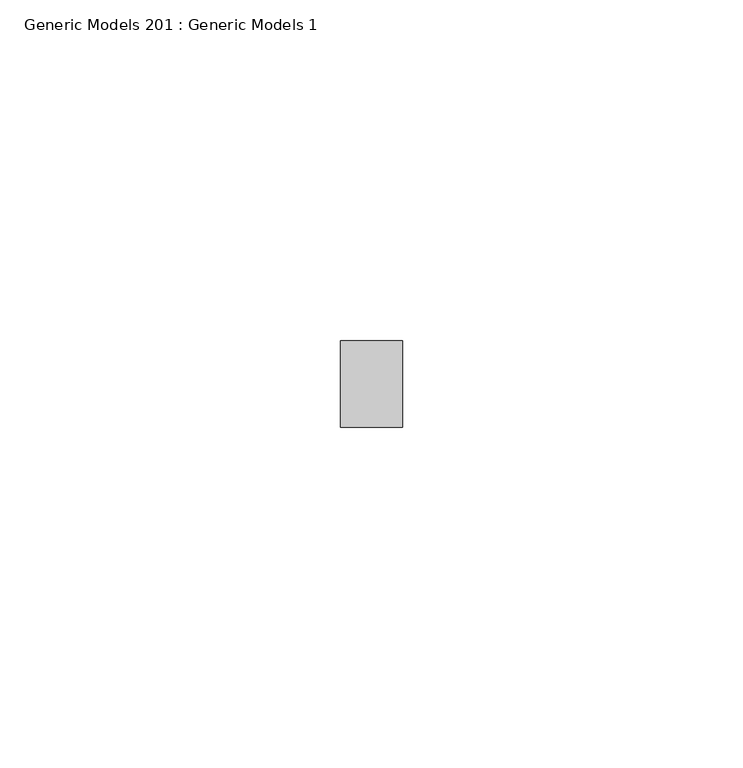
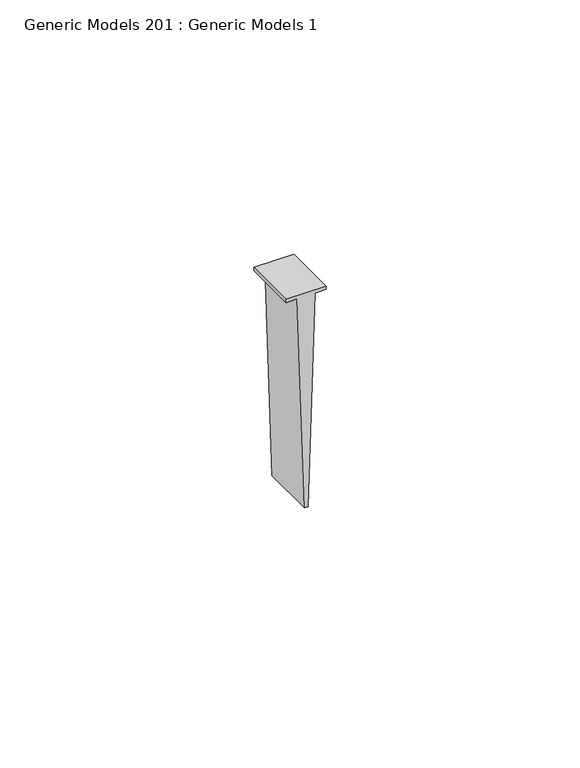
"""IFC4 building model written with IfcOpenShell, lengths in millimetres: proxy geometry, Generic Models 201 : Generic Models 1."""

import ifcopenshell
import ifcopenshell.guid

model = None  # the IFC model being written
_history = None  # IfcOwnerHistory: only IFC2X3 demands one
_inside = {}  # id of a spatial element -> (the spatial element, [elements in it])
_under = {}  # id of a project, library or spatial element -> (it, [spatial elements below it])
_declared = {}  # id of a project -> (the project, [libraries it declares])
_typed = {}  # id of a type object -> (the type object, [elements of that type])
_made_of = {}  # id of a material, layer set ... -> (it, [elements and type objects made of it])


def new_model(schema):
    """Start an empty IFC model of exactly this schema.

    Asked for "IFC4X3", IfcOpenShell would pick the latest addendum, in which some entities
    have other attributes; the version numbers below select the first issue.
    IFC2X3 requires an IfcOwnerHistory on every rooted entity: one is made here for all.
    """
    global model, _history
    if schema == "IFC4X3":
        model = ifcopenshell.file(schema_version=(4, 3, 0, 0))
    else:
        model = ifcopenshell.file(schema=schema)
    _inside.clear()
    _under.clear()
    _declared.clear()
    _typed.clear()
    _made_of.clear()
    _history = None
    if model.schema == "IFC2X3":
        org = make("IfcOrganization", Name="unknown")
        user = make(
            "IfcPersonAndOrganization",
            ThePerson=make("IfcPerson", FamilyName="unknown"),
            TheOrganization=org,
        )
        app = make(
            "IfcApplication",
            ApplicationDeveloper=org,
            Version="unknown",
            ApplicationFullName="unknown",
            ApplicationIdentifier="unknown",
        )
        _history = make(
            "IfcOwnerHistory",
            OwningUser=user,
            OwningApplication=app,
            ChangeAction="ADDED",
            CreationDate=0,
        )
    return model


def make(cls, **values):
    """One entity of the class cls with the attributes given. An attribute that is None is left unset."""
    return model.create_entity(
        cls, **{name: value for name, value in values.items() if value is not None}
    )


def rooted(cls, **values):
    """An entity with a GlobalId (a new one), such as an element, a storey or a relation."""
    return make(cls, GlobalId=ifcopenshell.guid.new(), OwnerHistory=_history, **values)


def si_unit(unit_type, name, prefix=None):
    """IfcSIUnit, for example si_unit("LENGTHUNIT", "METRE", prefix="MILLI")."""
    return make("IfcSIUnit", UnitType=unit_type, Prefix=prefix, Name=name)


def assignment(units):
    """IfcUnitAssignment: the units of a project."""
    return None if units is None else make("IfcUnitAssignment", Units=units)


def point(xyz):
    """IfcCartesianPoint."""
    return None if xyz is None else make("IfcCartesianPoint", Coordinates=xyz)


def direction(xyz):
    """IfcDirection."""
    return None if xyz is None else make("IfcDirection", DirectionRatios=xyz)


def frame(location, z_axis=None, x_axis=None):
    """IfcAxis2Placement3D, a coordinate frame: its origin and axes. An axis left out is left unset."""
    return make(
        "IfcAxis2Placement3D",
        Location=point(location),
        Axis=direction(z_axis),
        RefDirection=direction(x_axis),
    )


def origin():
    """The frame at (0, 0, 0) with its axes left unset."""
    return frame((0.0, 0.0, 0.0))


def place(relative_to, where):
    """IfcLocalPlacement: puts the frame where relative to a parent placement (None: the world)."""
    return make(
        "IfcLocalPlacement", PlacementRelTo=relative_to, RelativePlacement=where
    )


def context(
    kind, dimensions, precision=None, world=None, true_north=None, identifier=None
):
    """IfcGeometricRepresentationContext, for example the 3D "Model" context."""
    return make(
        "IfcGeometricRepresentationContext",
        ContextIdentifier=identifier,
        ContextType=kind,
        CoordinateSpaceDimension=dimensions,
        Precision=precision,
        WorldCoordinateSystem=world,
        TrueNorth=true_north,
    )


def project(units=None, contexts=None):
    """IfcProject with its units and contexts."""
    return rooted(
        "IfcProject",
        Name="project",
        RepresentationContexts=contexts,
        UnitsInContext=assignment(units),
    )


def spatial(cls, under=None, at=None, **own):
    """A site, building, storey or space (cls), placed at a placement, below another one or the project."""
    s = rooted(cls, ObjectPlacement=at, **own)
    if under is not None:
        _under.setdefault(under.id(), (under, []))[1].append(s)
    return s


def polyline(points):
    """IfcPolyline through the points."""
    return make("IfcPolyline", Points=[point(p) for p in points])


def outline(outer, holes=None, kind="AREA"):
    """IfcArbitraryClosedProfileDef: a profile drawn as a closed curve; with holes, ...WithVoids."""
    if holes is None:
        return make("IfcArbitraryClosedProfileDef", ProfileType=kind, OuterCurve=outer)
    return make(
        "IfcArbitraryProfileDefWithVoids",
        ProfileType=kind,
        OuterCurve=outer,
        InnerCurves=holes,
    )


def extrude(swept, where, along, depth):
    """IfcExtrudedAreaSolid: the profile swept, set in the frame where, extruded along a direction by depth."""
    return make(
        "IfcExtrudedAreaSolid",
        SweptArea=swept,
        Position=where,
        ExtrudedDirection=direction(along),
        Depth=depth,
    )


def shape(context_of_items, identifier, shape_type, items):
    """IfcShapeRepresentation: the items that make up one representation, for example the "Body"."""
    return make(
        "IfcShapeRepresentation",
        ContextOfItems=context_of_items,
        RepresentationIdentifier=identifier,
        RepresentationType=shape_type,
        Items=items,
    )


def source(mapping_origin, context_of_items, identifier, shape_type, items):
    """IfcRepresentationMap: a shape defined once, which mapped items show again and again."""
    return make(
        "IfcRepresentationMap",
        MappingOrigin=mapping_origin,
        MappedRepresentation=shape(context_of_items, identifier, shape_type, items),
    )


def transform(
    local_origin,
    x_axis=None,
    y_axis=None,
    z_axis=None,
    scale=None,
    scale2=None,
    scale3=None,
    uniform=True,
):
    """IfcCartesianTransformationOperator3D, or its non-uniform kind. x_axis, y_axis, z_axis: its Axis1, 2, 3."""
    if uniform:
        return make(
            "IfcCartesianTransformationOperator3D",
            Axis1=direction(x_axis),
            Axis2=direction(y_axis),
            LocalOrigin=point(local_origin),
            Scale=scale,
            Axis3=direction(z_axis),
        )
    return make(
        "IfcCartesianTransformationOperator3DnonUniform",
        Axis1=direction(x_axis),
        Axis2=direction(y_axis),
        LocalOrigin=point(local_origin),
        Scale=scale,
        Axis3=direction(z_axis),
        Scale2=scale2,
        Scale3=scale3,
    )


def mapped(mapping_source, mapping_target):
    """IfcMappedItem: shows the shape of a source again, moved by a transform."""
    return make(
        "IfcMappedItem", MappingSource=mapping_source, MappingTarget=mapping_target
    )


def made_of(thing, what):
    """Note that an element or type object is made of a material, layer set ...; save() writes the relation."""
    if what is not None:
        _made_of.setdefault(what.id(), (what, []))[1].append(thing)
    return thing


def element(
    cls,
    number,
    at=None,
    inside=None,
    cuts=None,
    type_object=None,
    material=None,
    context=None,
    identifier="Body",
    shape_type=None,
    held_by="IfcProductDefinitionShape",
    body=None,
    shapes=None,
    **own,
):
    """One element of the class cls, such as IfcWall. Its Tag is "e" and its number.

    at: its placement. inside: the storey or other place that contains it. cuts: it is an
    opening in that element (IfcRelVoidsElement). A single representation is given by context,
    identifier, shape_type and body (its items); several are given by shapes. held_by: the class
    of the entity that holds the representations. save() writes the other relations.
    """
    e = rooted(cls, Tag="e%d" % number, ObjectPlacement=at, **own)
    if body is not None:
        shapes = [shape(context, identifier, shape_type, body)]
    if shapes is not None:
        e.Representation = make(held_by, Representations=shapes)
    if inside is not None:
        _inside.setdefault(inside.id(), (inside, []))[1].append(e)
    if cuts is not None:
        rooted(
            "IfcRelVoidsElement", RelatingBuildingElement=cuts, RelatedOpeningElement=e
        )
    if type_object is not None:
        _typed.setdefault(type_object.id(), (type_object, []))[1].append(e)
    return made_of(e, material)


def aggregate(whole, parts):
    """IfcRelAggregates: a whole, such as a stair, and the parts it consists of."""
    return rooted("IfcRelAggregates", RelatingObject=whole, RelatedObjects=parts)


def save(model, path):
    """Write the relations noted so far, then the file.

    IfcRelAggregates (storeys below a building ...), IfcRelContainedInSpatialStructure (elements
    in a storey), IfcRelDefinesByType, IfcRelAssociatesMaterial and IfcRelDeclares: one each for
    every whole, place, type object, material and project.
    """
    for whole, parts in _under.values():
        aggregate(whole, parts)
    for where, things in _inside.values():
        rooted(
            "IfcRelContainedInSpatialStructure",
            RelatedElements=things,
            RelatingStructure=where,
        )
    for kind, things in _typed.values():
        rooted("IfcRelDefinesByType", RelatedObjects=things, RelatingType=kind)
    for what, things in _made_of.values():
        rooted("IfcRelAssociatesMaterial", RelatedObjects=things, RelatingMaterial=what)
    for by, libraries in _declared.values():
        rooted("IfcRelDeclares", RelatingContext=by, RelatedDefinitions=libraries)
    model.write(path)


def generic_models_201_generic_models_1_2740a068(model_context):
    return source(origin(), model_context, "Body", "SweptSolid", [
        extrude(outline(polyline([(-1922.0660706, 52599.8605108), (-1922.8598206, 52599.8605108), (-1922.8598206, 52602.4103744), (-1973.6598206, 52604.0077635), (-1973.6598206, 52604.8064581), (-1922.8598206, 52606.4038472), (-1922.8598206, 52608.9537108), (-1922.0660706, 52608.9537108), (-1922.0660706, 52599.8605108)])), frame((0.0, 565.15, 0.0), z_axis=(0.0, 1.0, 0.0), x_axis=(0.0, 0.0, 1.0)), (0.0, 0.0, 1.0), 12.7),
    ])


if __name__ == "__main__":
    model = new_model("IFC4")
    model_context = context("Model", 3, world=origin())
    ifc_project = project(units=[si_unit("LENGTHUNIT", "METRE", prefix="MILLI")], contexts=[model_context])
    site = spatial("IfcSite", under=ifc_project)
    building = spatial("IfcBuilding", under=site)
    placement = place(None, origin())
    generic_models_201_generic_models_1_shape = generic_models_201_generic_models_1_2740a068(model_context)
    element("IfcBuildingElementProxy", 1, Name="Generic Models 201 : Generic Models 1", ObjectType="Generic Models 201 : Generic Models 1", at=placement, inside=building, context=model_context, shape_type="MappedRepresentation", body=[
        mapped(generic_models_201_generic_models_1_shape, transform((0.0, 0.0, 0.0), x_axis=(1.0, 0.0, 0.0), y_axis=(0.0, 1.0, 0.0), z_axis=(0.0, 0.0, 1.0))),
    ])
    save(model, "model.ifc")

# Revit data of these elements
# Element 1 (IfcBuildingElementProxy, "Generic Models 201 : Generic Models 1")
#   Materials on its faces: "METAL RUNNER CHANNEL; FASTEN @ 24\" O.C."
# Materials
#   "METAL RUNNER CHANNEL; FASTEN @ 24\" O.C.": class "Unassigned", colour RGB 210 209 208, transparency 0, Keynote = "M05121300.02", Cost = 0
